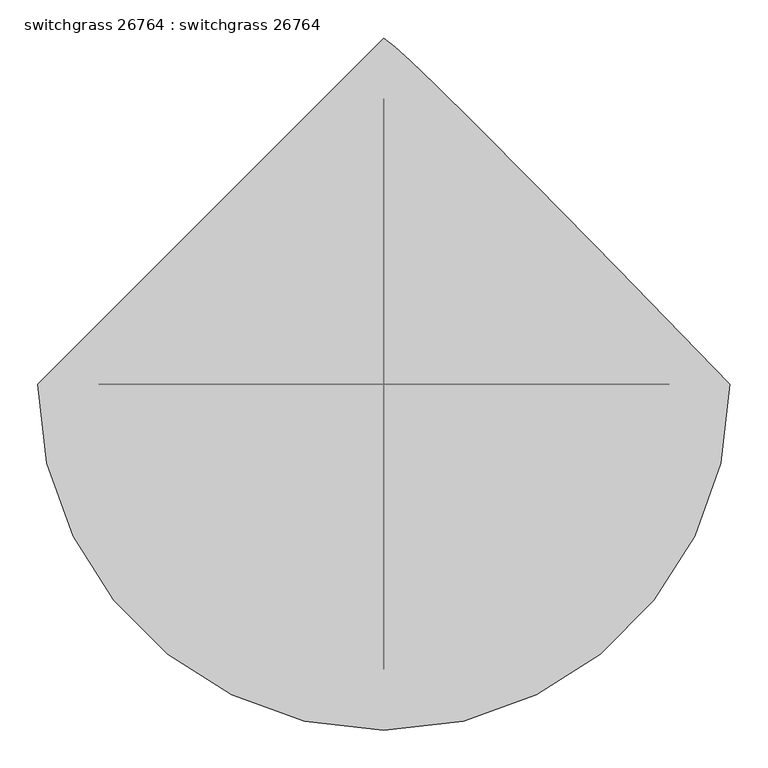
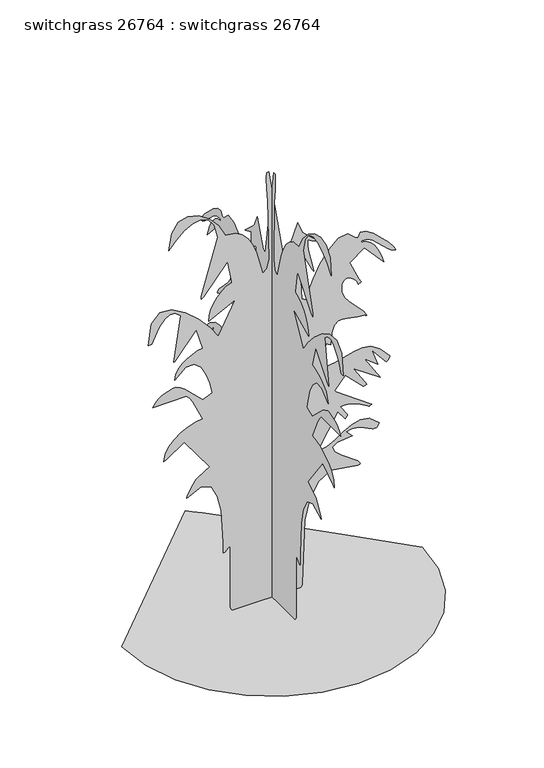
"""IFC4 building model written with IfcOpenShell, lengths in millimetres: proxy geometry, switchgrass 26764 : switchgrass 26764."""

from ifc_helpers import new_model, si_unit, origin, place, context, project, spatial, triangles, source, transform, mapped, element, save


def switchgrass_26764_switchgrass_26764_1323c538(model_context):
    return source(origin(), model_context, "Body", "Tessellation", [
        triangles([(-457.5348269, 0.0, 5.72e-05), (-445.4393443, -104.8366151, 5.72e-05), (-410.9893759, -201.1121793, 5.72e-05), (-356.9483794, -286.0697479, 5.72e-05), (-286.0697479, -356.9483794, 5.72e-05), (-201.1121793, -410.9893759, 5.72e-05), (-104.8366151, -445.4393443, 5.72e-05), (2e-05, -457.5348269, 5.72e-05), (104.8366151, -445.4393443, 5.72e-05), (201.1124336, -410.9893759, 5.72e-05), (286.0697479, -356.9483794, 5.72e-05), (356.9483794, -286.0697479, 5.72e-05), (410.9893759, -201.1121793, 5.72e-05), (445.4393443, -104.8366151, 5.72e-05), (457.5348269, 4e-05, 5.72e-05), (308.8459013, 152.5179615, 5.72e-05), (198.615602, 264.8099809, 5.72e-05), (120.4339824, 343.5803727, 5.72e-05), (67.8913365, 395.5334879, 5.72e-05), (34.5780016, 427.3748946, 5.72e-05), (14.0840831, 445.8076721, 5.72e-05), (-6e-05, 457.5348269, 5.72e-05), (34.93284, 5.5e-06, 1088.4574717), (36.237382, 5.5e-06, 1088.5946726), (37.9539129, 5.5e-06, 1088.9655075), (39.8896437, 5.5e-06, 1089.5065355), (41.8515379, 5.4e-06, 1090.1567139), (43.6465546, 5.4e-06, 1090.8526743), (45.0816551, 5.3e-06, 1091.5334467), (45.9643001, 5.3e-06, 1092.1353722), (79.0584374, 3e-07, 1176.7097157), (93.7670509, 2.4e-06, 1139.9381956), (141.570056, 5.1e-06, 1095.8133453), (139.9581813, 5e-06, 1096.2705122), (120.3097713, 3.5e-06, 1104.9699812), (109.4510318, 2.7e-06, 1111.5257584), (108.7718309, 3.8e-06, 1094.9344746), (110.1157441, 4.9e-06, 1079.5497305), (124.110375, 9.5e-06, 1020.4566805), (126.8614426, 1.06e-05, 1003.8832008), (124.028585, 1.03e-05, 1007.8913137), (90.0899044, 6.2e-06, 1077.4263136), (82.7355931, 6.2e-06, 1077.4263136), (90.0899044, 1.52e-05, 926.664731), (91.5981517, 1.52e-05, 926.3243448), (93.839948, 1.52e-05, 925.4277426), (96.493992, 1.53e-05, 924.1679358), (99.2384648, 1.54e-05, 922.7353924), (101.7517925, 1.55e-05, 921.3205805), (103.7124104, 1.55e-05, 920.1165842), (104.7985178, 1.56e-05, 919.30893), (110.3578079, 1.41e-05, 944.2085003), (125.3806282, 1.19e-05, 981.1629307), (147.3843723, 9.5e-06, 1022.163553), (173.8869515, 7.3e-06, 1059.1942142), (202.4055415, 5.8e-06, 1084.2512604), (230.4577718, 5.5e-06, 1089.3210817), (255.5618354, 6.8e-06, 1066.3950829), (262.9151293, 6.8e-06, 1066.3950829), (269.3514915, 6.1e-06, 1080.2456909), (285.9199024, 6.4e-06, 1077.2713085), (308.5106383, 7.4e-06, 1062.4834757), (355.3227882, 1.03e-05, 1017.5331671), (371.3222114, 1.13e-05, 997.3934807), (376.9076989, 1.17e-05, 985.4987125), (366.3362148, 1.13e-05, 987.6501074), (353.3212752, 1.07e-05, 997.467168), (306.0061764, 8.2e-06, 1041.5234179), (289.6028898, 7.7e-06, 1050.6166128), (273.9463418, 7.7e-06, 1051.6859516), (270.2709666, 7.9e-06, 1048.0105946), (286.0621357, 8.1e-06, 1044.6704641), (300.011793, 8.7e-06, 1035.6788618), (312.0590046, 9.4e-06, 1022.5750105), (322.1529742, 1.04e-05, 1006.8905754), (330.2352207, 1.14e-05, 990.169721), (336.2473901, 1.23e-05, 973.9468014), (340.1361425, 1.32e-05, 959.7583506), (281.3021792, 9.2e-06, 1025.9481331), (237.175821, 1.12e-05, 992.8519701), (237.8959079, 1.14e-05, 989.6693882), (264.7083701, 1.53e-05, 931.0716568), (271.2971213, 1.6e-05, 919.3597263), (262.201401, 1.58e-05, 915.7986065), (257.5227259, 1.51e-05, 925.7833895), (250.3543407, 1.46e-05, 934.7876364), (241.7117542, 1.42e-05, 941.820928), (232.6099115, 1.39e-05, 945.8899384), (224.0638488, 1.4e-05, 946.014422), (217.0887659, 1.43e-05, 941.1985823), (212.6996442, 1.49e-05, 930.4569414), (212.5952538, 1.63e-05, 907.9474869), (220.1395426, 1.74e-05, 888.4809425), (232.934274, 1.85e-05, 871.1581627), (278.8409195, 2.13e-05, 823.0557209), (288.6554731, 2.24e-05, 805.3188675), (284.9775544, 2.24e-05, 805.3188675), (284.9775544, 2.22e-05, 808.9968407), (261.1244319, 2.2e-05, 811.3030952), (219.0793602, 2.16e-05, 819.2355326), (202.3661725, 2.16e-05, 817.8461552), (189.5122514, 2.22e-05, 808.2093887), (181.2572684, 2.35e-05, 786.8149824), (178.341349, 2.57e-05, 750.1603157), (163.6327264, 2.52e-05, 757.5161167), (156.2784152, 2.96e-05, 683.9730766), (191.325313, 2.94e-05, 687.4935013), (248.5903132, 2.85e-05, 703.0763437), (274.1444584, 2.83e-05, 706.7441431), (299.8746466, 2.85e-05, 702.0628881), (327.443785, 2.96e-05, 684.8417009), (358.5206308, 3.16e-05, 650.8794571), (358.1040865, 3.17e-05, 648.5070728), (356.9788645, 3.19e-05, 645.8020054), (355.3380126, 3.21e-05, 643.0156202), (353.374615, 3.22e-05, 640.4019716), (351.2841903, 3.24e-05, 638.2225988), (349.2598226, 3.24e-05, 636.7265419), (347.4894364, 3.25e-05, 636.1703259), (303.3646043, 2.94e-05, 687.6509771), (321.6983145, 3.25e-05, 637.1100941), (281.4164709, 3.05e-05, 668.6899252), (329.1049481, 3.51e-05, 592.0454756), (248.2070336, 3.18e-05, 647.2014839), (249.7422051, 3.2e-05, 643.9071356), (282.1810136, 3.5e-05, 593.8082314), (288.6554731, 3.55e-05, 584.6896382), (287.7740952, 3.56e-05, 584.486453), (278.9298131, 3.57e-05, 581.2174664), (277.6242605, 3.58e-05, 581.0117014), (222.4671985, 3.25e-05, 636.1703259), (189.3728159, 3.49e-05, 595.7208326), (303.3646043, 3.97e-05, 514.8244623), (302.6254598, 3.97e-05, 514.6872977), (301.5739069, 3.97e-05, 514.3164628), (300.3369185, 3.98e-05, 513.7754348), (299.0364347, 3.98e-05, 513.1252201), (297.7994644, 3.98e-05, 512.4292597), (296.7479115, 3.99e-05, 511.7485236), (296.008767, 3.99e-05, 511.1465618), (285.8436898, 3.91e-05, 517.9918562), (258.9959281, 3.82e-05, 530.9178841), (230.2492453, 3.8e-05, 539.6935839), (217.7123288, 3.81e-05, 541.3522036), (207.7585759, 3.82e-05, 540.564788), (229.8212554, 4.01e-05, 507.4711684), (229.5405858, 4.03e-05, 505.7007823), (228.7854538, 4.04e-05, 503.6738711), (227.6866473, 4.05e-05, 501.5834464), (226.3747361, 4.06e-05, 499.6225923), (224.9802718, 4.07e-05, 497.9817404), (223.6343329, 4.08e-05, 496.8565184), (222.4671985, 4.08e-05, 496.4374306), (200.4042828, 3.9e-05, 525.8556567), (137.8929095, 4.54e-05, 419.2189608), (166.0807783, 4.51e-05, 424.9746051), (192.3560459, 4.44e-05, 438.7921846), (217.6356256, 4.35e-05, 455.4799742), (242.8367037, 4.28e-05, 469.858893), (268.8765023, 4.25e-05, 476.7397593), (296.6716989, 4.29e-05, 470.9409127), (327.1389708, 4.44e-05, 447.2757874), (326.9992627, 4.44e-05, 446.6026817), (318.6350567, 4.45e-05, 435.0634515), (318.0737174, 4.45e-05, 433.928092), (304.8454187, 4.44e-05, 435.7644988), (292.8515469, 4.41e-05, 440.3060094), (269.6842292, 4.35e-05, 451.6369311), (257.0629792, 4.32e-05, 455.5028289), (242.7904856, 4.32e-05, 456.2140137), (226.1443541, 4.34e-05, 452.3125803), (244.5298779, 4.45e-05, 433.928092), (198.3082625, 4.53e-05, 429.3560964), (183.5841612, 4.73e-05, 417.3698367), (191.3966749, 5e-05, 400.5525129), (212.7859943, 5.3e-05, 381.4872886), (260.4513443, 5.75e-05, 346.9661762), (268.8053947, 5.81e-05, 336.6766517), (266.5219404, 5.8e-05, 334.0198371), (261.1066641, 5.8e-05, 333.3340141), (178.1579663, 6e-05, 346.4759809), (140.1265758, 6.16e-05, 322.2393062), (114.9013532, 6.35e-05, 274.7464384), (99.9910624, 6.53e-05, 212.9973368), (92.4787665, 7.02e-05, 12.5836557), (91.8127825, 7.03e-05, 8.321819), (90.5290672, 7.04e-05, 4.9722738), (88.4818266, 7.04e-05, 2.3959441), (85.5242583, 7.04e-05, 0.4537325), (-118.3633693, 7.08e-05, 2.4e-05), (-122.0969169, 7.09e-05, 2.3783469), (-124.6485962, 7.1e-05, 5.1976728), (-126.2274606, 7.11e-05, 8.3395482), (-127.0420366, 7.12e-05, 11.6852833), (-127.3018772, 7.12e-05, 15.1165158), (-126.9912402, 7.13e-05, 21.7608447), (-126.8614426, 5.81e-05, 205.9442608), (-129.3712185, 5.82e-05, 207.0623793), (-132.5175108, 5.83e-05, 205.407811), (-143.2413748, 5.85e-05, 195.0563171), (-146.3985949, 5.86e-05, 193.5589884), (-148.9243673, 5.88e-05, 194.9127939), (-148.7935613, 5.68e-05, 227.8207598), (-154.894379, 5.06e-05, 331.9700349), (-165.8895291, 4.76e-05, 382.8233262), (-185.3575813, 4.54e-05, 419.2723005), (-215.6798221, 4.47e-05, 431.1264825), (-259.2397541, 4.61e-05, 408.1877664), (-259.6156759, 4.59e-05, 410.1283092), (-257.8935608, 4.56e-05, 415.3124405), (-244.622078, 4.41e-05, 440.6336783), (-233.4986654, 4.32e-05, 455.9905171), (-232.2906359, 4.31e-05, 458.4568274), (-228.0976142, 4.28e-05, 462.3633476), (-205.3272926, 4.19e-05, 477.5550802), (-189.3728159, 4.15e-05, 485.4061998), (-266.593048, 3.51e-05, 592.0454756), (-321.7491108, 3.73e-05, 555.2739192), (-329.1049481, 3.75e-05, 551.5960187), (-325.1247405, 3.62e-05, 573.5644452), (-314.238341, 3.5e-05, 593.5542134), (-298.0255225, 3.4e-05, 611.0903887), (-278.058609, 3.31e-05, 625.6979273), (-255.9199894, 3.24e-05, 636.9018219), (-233.1864933, 3.2e-05, 644.2271742), (-211.4357316, 3.18e-05, 647.2014839), (-213.7123368, 3.13e-05, 653.8029705), (-240.9860717, 2.74e-05, 712.3753401), (-250.6378082, 2.7e-05, 726.9625311), (-260.7383544, 2.74e-05, 738.2883659), (-362.9504113, 3.12e-05, 737.0260157), (-353.9791203, 3.02e-05, 749.4745291), (-345.6987391, 2.91e-05, 758.1181149), (-337.7028245, 2.78e-05, 763.9169615), (-329.5900566, 2.65e-05, 767.8437567), (-300.461384, 2.23e-05, 778.026638), (-293.1055467, 2.23e-05, 778.026638), (-278.8536186, 2.33e-05, 770.8663919), (-266.2755528, 2.42e-05, 762.6672558), (-211.4357316, 2.81e-05, 709.7133659), (-182.0185046, 2.74e-05, 720.7445967), (-189.8899537, 2.53e-05, 755.5907982), (-200.3534683, 2.34e-05, 786.4390606), (-215.7232605, 2.17e-05, 814.9480036), (-236.4161108, 2.06e-05, 832.6416183), (-262.8490904, 2.07e-05, 831.0515991), (-295.4347286, 2.24e-05, 801.707024), (-292.5975471, 2.14e-05, 818.2246204), (-284.8327776, 2.06e-05, 832.9972652), (-273.265624, 1.99e-05, 845.8724968), (-259.0162394, 1.93e-05, 856.6852816), (-243.2146603, 1.88e-05, 865.2806145), (-226.9795139, 1.84e-05, 871.5010923), (-211.4357316, 1.82e-05, 875.1840797), (-229.8215097, 1.43e-05, 941.3738623), (-296.0113104, 1.91e-05, 860.4749485), (-299.6866857, 1.91e-05, 860.4749485), (-277.7029984, 1e-05, 1003.3269121), (-294.71337, 9.2e-06, 1017.2435772), (-311.0531794, 9.3e-06, 1017.8481188), (-326.2398251, 9.9e-06, 1008.5745569), (-339.7957927, 1.1e-05, 992.857057), (-351.2410243, 1.22e-05, 974.1270956), (-365.8764682, 1.43e-05, 941.3738623), (-376.9076989, 1.43e-05, 941.3738623), (-367.2226796, 1.04e-05, 1007.1064779), (-341.7211112, 8.7e-06, 1034.375889), (-305.7369704, 8.9e-06, 1031.8511158), (-264.604234, 1.03e-05, 1008.203722), (-223.6538811, 1.25e-05, 972.1078148), (-188.2191436, 1.48e-05, 932.229871), (-163.6329808, 1.69e-05, 897.2464685), (-112.1528291, 1.1e-05, 996.5298706), (-193.0499715, 1.34e-05, 956.0804501), (-191.1398955, 1.24e-05, 973.1822405), (-185.7319771, 1.13e-05, 990.7996971), (-177.3111248, 1.03e-05, 1008.0386158), (-166.3611936, 9.4e-06, 1024.0076265), (-153.3675827, 8.5e-06, 1037.8124525), (-138.8136563, 7.9e-06, 1048.5617237), (-123.1842869, 7.5e-06, 1055.3638521), (-122.7161651, 7.3e-06, 1058.0105656), (-134.2157538, 3.3e-06, 1125.2290644), (-138.2424067, 3.4e-06, 1124.548292), (-207.9053874, 8.4e-06, 1039.524412), (-215.1128872, 8.8e-06, 1033.3014633), (-214.9937629, 6.5e-06, 1043.3674913), (-165.5864953, -2.1e-06, 1216.2397156), (-176.4513299, -4.6e-06, 1258.3223213), (-194.0382833, -6.1e-06, 1282.2669353), (-216.3737477, -6.6e-06, 1290.7911243), (-241.4831526, -6.4e-06, 1286.6001011), (-267.3931445, -5.6e-06, 1272.4143391), (-292.1276449, -4.3e-06, 1250.938615), (-313.7150808, -2.8e-06, 1224.8909317), (-305.8919028, -5.9e-06, 1277.1868675), (-285.2950496, -7.5e-06, 1305.4849949), (-256.2374846, -8e-06, 1313.3996281), (-223.0242321, -7.4e-06, 1304.5427559), (-189.9694546, -6.1e-06, 1282.5285473), (-161.3812832, -4.2e-06, 1250.9716072), (-141.570056, -1.9e-06, 1213.4812357), (-111.003735, -1.7e-06, 1210.2630455), (-90.0827918, -1e-06, 1197.192259), (-72.9868286, 2e-07, 1178.0406664), (-59.2218167, 1.6e-06, 1154.5431181), (-48.2927191, 3.1e-06, 1128.4294504), (-27.578531, 7.7e-06, 1051.6859516), (-15.6259369, 7e-06, 1062.9330849), (-8.9939533, 5.3e-06, 1092.3284563), (-12.8700152, -6.1e-06, 1283.3463753), (-14.1246216, -5.9e-06, 1292.5767712), (-15.1875847, -6.3e-06, 1303.493692), (-16.0281459, -7e-06, 1315.7644547), (-16.6151389, -8.1e-06, 1329.0460567), (-16.9180092, -9.2e-06, 1343.0058151), (-16.9057404, -1.04e-05, 1357.3034889), (-16.5471686, -1.14e-05, 1371.5986919), (-9.1928857, -1.14e-05, 1371.5986919), (-3.16e-05, 34.93284, 1088.4574717), (-3.16e-05, 36.237382, 1088.5946726), (-3.16e-05, 37.9539129, 1088.9655075), (-3.16e-05, 39.8896437, 1089.509079), (-3.16e-05, 41.8515379, 1090.1567139), (-3.16e-05, 43.6465546, 1090.8552177), (-3.16e-05, 45.0819049, 1091.5334467), (-3.16e-05, 45.9643001, 1092.1353722), (-3.16e-05, 79.0586918, 1176.7097157), (-3.16e-05, 93.7673053, 1139.9381956), (-3.16e-05, 141.570056, 1095.8133453), (-3.15e-05, 139.9581813, 1096.2705122), (-3.05e-05, 120.3097713, 1104.9699812), (-3.01e-05, 109.4512861, 1111.5257584), (-3.02e-05, 108.7720852, 1094.9344746), (-3.04e-05, 110.1157441, 1079.5497305), (-3.15e-05, 124.1106294, 1020.4566805), (-3.16e-05, 126.8614426, 1003.8832008), (-3.16e-05, 124.028585, 1007.8913137), (-3.16e-05, 90.0901496, 1077.4263136), (-3.16e-05, 82.7358474, 1077.4263136), (-3.16e-05, 90.0901496, 926.664731), (-3.16e-05, 91.5981517, 926.3243448), (-3.16e-05, 93.8402023, 925.4277426), (-3.16e-05, 96.493992, 924.1679358), (-3.16e-05, 99.2387191, 922.7353924), (-3.16e-05, 101.7517925, 921.3205805), (-3.16e-05, 103.7124104, 920.1165842), (-3.16e-05, 104.7985178, 919.30893), (-3.16e-05, 110.3578079, 944.2085003), (-3.16e-05, 125.3806282, 981.1629307), (-3.16e-05, 147.3846266, 1022.163553), (-3.16e-05, 173.8872059, 1059.1942142), (-3.16e-05, 202.4055415, 1084.2512604), (-3.16e-05, 230.4580261, 1089.3210817), (-3.16e-05, 255.5618354, 1066.3950829), (-3.16e-05, 262.9151293, 1066.3950829), (-3.16e-05, 269.3514915, 1080.2456909), (-3.18e-05, 285.9199024, 1077.2713085), (-3.19e-05, 308.5106383, 1062.4834757), (-3.21e-05, 355.3227882, 1017.5331671), (-3.19e-05, 371.3222114, 997.3934807), (-3.16e-05, 376.9076989, 985.4987125), (-3.14e-05, 366.3362148, 987.6501074), (-3.13e-05, 353.3212752, 997.467168), (-3.14e-05, 306.0061764, 1041.5234179), (-3.15e-05, 289.6028898, 1050.6166128), (-3.16e-05, 273.9463418, 1051.6859516), (-3.16e-05, 270.2709666, 1048.0105946), (-3.16e-05, 286.0621357, 1044.6704641), (-3.16e-05, 300.011793, 1035.6788618), (-3.16e-05, 312.0590046, 1022.5750105), (-3.16e-05, 322.1529742, 1006.8905754), (-3.16e-05, 330.2352207, 990.169721), (-3.16e-05, 336.2473901, 973.9468014), (-3.16e-05, 340.1361425, 959.7583506), (-3.16e-05, 281.3021792, 1025.9481331), (-3.16e-05, 237.175821, 992.8519701), (-3.16e-05, 237.8959079, 989.6693882), (-3.19e-05, 264.7083701, 931.0716568), (-3.19e-05, 271.2971213, 919.3597263), (-3.16e-05, 262.201401, 915.7986065), (-3.15e-05, 257.5227259, 925.7833895), (-3.15e-05, 250.3543407, 934.7876364), (-3.15e-05, 241.7117542, 941.820928), (-3.15e-05, 232.6099115, 945.8924818), (-3.15e-05, 224.0641032, 946.014422), (-3.15e-05, 217.0887659, 941.1985823), (-3.16e-05, 212.6996442, 930.4569414), (-3.16e-05, 212.5955081, 907.9474869), (-3.16e-05, 220.1397969, 888.4809425), (-3.16e-05, 232.934274, 871.1581627), (-3.16e-05, 278.8409195, 823.0557209), (-3.16e-05, 288.6554731, 805.3188675), (-3.16e-05, 284.9775544, 805.3188675), (-3.16e-05, 284.9775544, 808.9968407), (-3.16e-05, 261.1244319, 811.3030952), (-3.16e-05, 219.0796145, 819.2355326), (-3.16e-05, 202.3661725, 817.8461552), (-3.16e-05, 189.5122514, 808.2093887), (-3.16e-05, 181.2575227, 786.8149824), (-3.16e-05, 178.3416033, 750.1603157), (-3.16e-05, 163.6329808, 757.5161167), (-3.16e-05, 156.2786695, 683.9730766), (-3.16e-05, 191.325313, 687.4935013), (-3.16e-05, 248.5905676, 703.0763437), (-3.16e-05, 274.1444584, 706.7441431), (-3.16e-05, 299.8746466, 702.0628881), (-3.16e-05, 327.443785, 684.8417009), (-3.16e-05, 358.5206308, 650.8794571), (-3.16e-05, 358.1040865, 648.5070728), (-3.16e-05, 356.9788645, 645.8020054), (-3.16e-05, 355.3380126, 643.0156202), (-3.16e-05, 353.374615, 640.4019716), (-3.16e-05, 351.2841903, 638.2225988), (-3.16e-05, 349.2598226, 636.7265419), (-3.16e-05, 347.4894364, 636.1703259), (-3.16e-05, 303.3646043, 687.6509771), (-3.17e-05, 321.6983145, 637.1100941), (-3.16e-05, 281.4164709, 668.6899252), (-3.16e-05, 329.1049481, 592.0454756), (-3.16e-05, 248.2072879, 647.2014839), (-3.16e-05, 249.7422051, 643.9071356), (-3.16e-05, 282.1810136, 593.8082314), (-3.16e-05, 288.6554731, 584.6896382), (-3.16e-05, 287.7740952, 584.486453), (-3.16e-05, 278.9298131, 581.2174664), (-3.16e-05, 277.6242605, 581.0117014), (-3.16e-05, 222.4671985, 636.1703259), (-3.16e-05, 189.3728159, 595.7208326), (-3.16e-05, 303.3646043, 514.8244623), (-3.16e-05, 302.6254598, 514.6872977), (-3.16e-05, 301.5739069, 514.3164628), (-3.16e-05, 300.3369185, 513.7754348), (-3.16e-05, 299.0364347, 513.1252201), (-3.16e-05, 297.7994644, 512.4292597), (-3.16e-05, 296.7479115, 511.7485236), (-3.16e-05, 296.0113104, 511.1465618), (-3.12e-05, 285.8436898, 517.9918562), (-3.1e-05, 258.9959281, 530.9178841), (-3.13e-05, 230.2494996, 539.6935839), (-3.15e-05, 217.7125832, 541.3522036), (-3.16e-05, 207.7585759, 540.564788), (-3.16e-05, 229.8215097, 507.4711684), (-3.16e-05, 229.5408401, 505.7007823), (-3.16e-05, 228.7857081, 503.6738711), (-3.16e-05, 227.6866473, 501.5834464), (-3.16e-05, 226.3747361, 499.6225923), (-3.16e-05, 224.9805262, 497.9817404), (-3.16e-05, 223.6343329, 496.8565184), (-3.16e-05, 222.4671985, 496.4374306), (-3.16e-05, 200.4042828, 525.8556567), (-3.16e-05, 137.8929095, 419.2189608), (-3.16e-05, 166.0807783, 424.9771485), (-3.17e-05, 192.3560459, 438.7921846), (-3.18e-05, 217.63588, 455.4799742), (-3.19e-05, 242.8367037, 469.858893), (-3.21e-05, 268.8765023, 476.7397593), (-3.21e-05, 296.6716989, 470.9409127), (-3.22e-05, 327.1389708, 447.2757874), (-3.21e-05, 326.9992627, 446.6026817), (-3.16e-05, 318.6350567, 435.0634515), (-3.16e-05, 318.0737174, 433.928092), (-3.16e-05, 304.8454187, 435.7644988), (-3.16e-05, 292.8540904, 440.3060094), (-3.16e-05, 269.6842292, 451.6369311), (-3.16e-05, 257.0629792, 455.5028289), (-3.16e-05, 242.7904856, 456.2140137), (-3.16e-05, 226.1443541, 452.3125803), (-3.16e-05, 244.5301323, 433.928092), (-3.21e-05, 198.3082625, 429.3560964), (-3.33e-05, 183.5841612, 417.3698367), (-3.51e-05, 191.3969293, 400.5525129), (-3.69e-05, 212.7862487, 381.4872886), (-3.94e-05, 260.4513443, 346.9661762), (-3.94e-05, 268.8053947, 336.6766517), (-3.91e-05, 266.5219404, 334.0198371), (-3.91e-05, 261.1066641, 333.3340141), (-4.18e-05, 178.1579663, 346.4759809), (-4.2e-05, 140.1265758, 322.2393062), (-4.1e-05, 114.9013532, 274.7464384), (-3.92e-05, 99.9910624, 212.9973368), (-3.21e-05, 92.4787665, 12.5836296), (-3.2e-05, 91.8127825, 8.3217934), (-3.19e-05, 90.5293216, 4.9722483), (-3.18e-05, 88.4818266, 2.3959185), (-3.16e-05, 85.5242583, 0.4537071), (-3.19e-05, -118.3631241, 0.0), (-3.22e-05, -122.0966625, 2.378324), (-3.24e-05, -124.6483418, 5.1976479), (-3.27e-05, -126.2272062, 8.3395226), (-3.3e-05, -127.0420366, 11.6852833), (-3.33e-05, -127.3018772, 15.1164896), (-3.38e-05, -126.9912402, 21.7608197), (-3.16e-05, -126.8614426, 205.9442608), (-3.17e-05, -129.3709642, 207.062125), (-3.17e-05, -132.5175108, 205.407811), (-3.13e-05, -143.2413748, 195.0563171), (-3.13e-05, -146.3985949, 193.5589884), (-3.16e-05, -148.924113, 194.9127939), (-3.16e-05, -148.7935613, 227.8207598), (-3.16e-05, -154.8941247, 331.9700349), (-3.16e-05, -165.8895291, 382.8233262), (-3.16e-05, -185.357327, 419.274844), (-3.16e-05, -215.6798221, 431.1264825), (-3.16e-05, -259.2397541, 408.1877664), (-3.16e-05, -259.6156759, 410.1283092), (-3.16e-05, -257.8935608, 415.3124405), (-3.16e-05, -244.6218236, 440.6336783), (-3.16e-05, -233.498411, 455.9905171), (-3.16e-05, -232.2906359, 458.4568274), (-3.16e-05, -228.0976142, 462.3658911), (-3.16e-05, -205.3272926, 477.5550802), (-3.16e-05, -189.3728159, 485.4061998), (-3.16e-05, -266.593048, 592.0454756), (-3.16e-05, -321.7491108, 555.2739192), (-3.16e-05, -329.1049481, 551.5960187), (-3.16e-05, -325.1247405, 573.5644452), (-3.16e-05, -314.238341, 593.5542134), (-3.16e-05, -298.0229791, 611.0903887), (-3.16e-05, -278.058609, 625.6979273), (-3.16e-05, -255.9199894, 636.9018219), (-3.16e-05, -233.186239, 644.2271742), (-3.16e-05, -211.4357316, 647.2014839), (-3.14e-05, -213.7123368, 653.8029705), (-3.1e-05, -240.9858174, 712.3753401), (-3.15e-05, -250.6378082, 726.9625311), (-3.26e-05, -260.7383544, 738.2883659), (-3.63e-05, -362.9504113, 737.0260157), (-3.61e-05, -353.9765768, 749.4745291), (-3.54e-05, -345.6987391, 758.1181149), (-3.45e-05, -337.7028245, 763.9169615), (-3.34e-05, -329.5900566, 767.8437567), (-2.99e-05, -300.461384, 778.026638), (-2.99e-05, -293.1055467, 778.026638), (-3.04e-05, -278.8536186, 770.8663919), (-3.08e-05, -266.2730093, 762.6672558), (-3.16e-05, -211.4357316, 709.7133659), (-3.16e-05, -182.0185046, 720.7445967), (-3.15e-05, -189.8899537, 755.5907982), (-3.15e-05, -200.353214, 786.4390606), (-3.15e-05, -215.7232605, 814.9480036), (-3.14e-05, -236.4161108, 832.6416183), (-3.14e-05, -262.8465652, 831.0515991), (-3.14e-05, -295.4347286, 801.707024), (-3.14e-05, -292.5975471, 818.2246204), (-3.14e-05, -284.8327776, 832.9972652), (-3.15e-05, -273.265624, 845.8724968), (-3.15e-05, -259.0162394, 856.6852816), (-3.15e-05, -243.2146603, 865.2806145), (-3.16e-05, -226.9795139, 871.5010923), (-3.16e-05, -211.4357316, 875.1840797), (-3.16e-05, -229.8212554, 941.3738623), (-3.16e-05, -296.008767, 860.4749485), (-3.16e-05, -299.6866857, 860.4749485), (-3.1e-05, -277.7029984, 1003.3269121), (-3.1e-05, -294.71337, 1017.2435772), (-3.11e-05, -311.0531794, 1017.8481188), (-3.12e-05, -326.2398251, 1008.5745569), (-3.13e-05, -339.7957927, 992.857057), (-3.14e-05, -351.2384809, 974.1270956), (-3.16e-05, -365.8764682, 941.3738623), (-3.16e-05, -376.9076989, 941.3738623), (-3.16e-05, -367.2226796, 1007.1064779), (-3.16e-05, -341.7211112, 1034.375889), (-3.16e-05, -305.7369704, 1031.8511158), (-3.16e-05, -264.604234, 1008.203722), (-3.16e-05, -223.6538811, 972.1078148), (-3.16e-05, -188.2191436, 932.229871), (-3.16e-05, -163.6327264, 897.2464685), (-3.16e-05, -112.1528291, 996.5298706), (-3.16e-05, -193.0499715, 956.0804501), (-3.16e-05, -191.1396412, 973.1822405), (-3.16e-05, -185.7317227, 990.7996971), (-3.16e-05, -177.3108705, 1008.0386158), (-3.16e-05, -166.3611936, 1024.0076265), (-3.16e-05, -153.3673283, 1037.8124525), (-3.16e-05, -138.813402, 1048.5617237), (-3.16e-05, -123.1842869, 1055.3638521), (-3.16e-05, -122.7159107, 1058.0105656), (-3.16e-05, -134.2157538, 1125.2290644), (-3.16e-05, -138.2424067, 1124.548292), (-3.16e-05, -207.9053874, 1039.524412), (-3.16e-05, -215.1128872, 1033.3014633), (-2.99e-05, -214.9935086, 1043.3674913), (-3.16e-05, -165.5864953, 1216.2397156), (-3.16e-05, -176.4510756, 1258.3223213), (-3.15e-05, -194.0382833, 1282.2669353), (-3.15e-05, -216.3737477, 1290.7911243), (-3.15e-05, -241.4828982, 1286.6001011), (-3.14e-05, -267.3931445, 1272.4143391), (-3.14e-05, -292.1276449, 1250.938615), (-3.14e-05, -313.7150808, 1224.8909317), (-3.14e-05, -305.8919028, 1277.1868675), (-3.14e-05, -285.2950496, 1305.4849949), (-3.15e-05, -256.2349411, 1313.3996281), (-3.15e-05, -223.0242321, 1304.5427559), (-3.15e-05, -189.9694546, 1282.5285473), (-3.16e-05, -161.3812832, 1250.9716072), (-3.16e-05, -141.570056, 1213.4812357), (-3.16e-05, -111.003735, 1210.2630455), (-3.16e-05, -90.0825374, 1197.192259), (-3.16e-05, -72.9865742, 1178.0432098), (-3.16e-05, -59.2215669, 1154.5431181), (-3.16e-05, -48.2927191, 1128.4294504), (-3.16e-05, -27.578531, 1051.6859516), (-3.16e-05, -15.6258108, 1062.9330849), (-3.16e-05, -8.9938517, 1092.3284563), (-3.16e-05, -12.869888, 1283.3463753), (-3.23e-05, -14.1245194, 1292.5767712), (-3.26e-05, -15.1874576, 1303.493692), (-3.26e-05, -16.0280449, 1315.7644547), (-3.23e-05, -16.6150378, 1329.0460567), (-3.2e-05, -16.917907, 1343.0058151), (-3.17e-05, -16.9056394, 1357.3034889), (-3.16e-05, -16.5470675, 1371.5986919), (-3.16e-05, -9.1927591, 1371.5986919)], [[21, 22, 1], [20, 21, 1], [19, 20, 1], [18, 19, 1], [17, 18, 1], [17, 1, 2], [17, 2, 3], [17, 3, 4], [16, 17, 4], [16, 4, 5], [16, 5, 6], [16, 6, 7], [16, 7, 8], [16, 8, 9], [16, 9, 10], [16, 10, 11], [16, 11, 12], [15, 16, 12], [14, 15, 12], [13, 14, 12], [122, 123, 124], [39, 40, 41], [77, 78, 79], [76, 77, 79], [32, 33, 34], [32, 34, 35], [32, 35, 36], [75, 76, 79], [294, 295, 296], [120, 121, 122], [74, 75, 79], [246, 247, 248], [246, 248, 249], [73, 74, 79], [30, 31, 32], [132, 133, 134], [285, 286, 287], [171, 172, 173], [246, 249, 250], [218, 219, 220], [64, 65, 66], [230, 231, 232], [230, 232, 233], [230, 233, 234], [230, 234, 235], [132, 134, 135], [230, 235, 236], [230, 236, 237], [230, 237, 238], [230, 238, 239], [273, 274, 275], [273, 275, 276], [273, 276, 277], [132, 135, 136], [72, 73, 79], [132, 136, 137], [273, 277, 278], [132, 137, 138], [217, 218, 220], [217, 220, 221], [217, 221, 222], [217, 222, 223], [126, 127, 128], [103, 104, 105], [229, 230, 239], [229, 239, 240], [132, 138, 139], [207, 208, 209], [207, 209, 210], [207, 210, 211], [273, 278, 279], [30, 32, 36], [30, 36, 37], [228, 229, 240], [293, 294, 296], [293, 296, 297], [293, 297, 298], [292, 293, 298], [292, 298, 299], [291, 292, 299], [291, 299, 300], [290, 291, 300], [289, 290, 300], [289, 300, 301], [288, 289, 301], [288, 301, 302], [132, 139, 140], [132, 140, 141], [132, 141, 142], [132, 142, 143], [132, 143, 144], [132, 144, 145], [64, 66, 67], [63, 64, 67], [256, 257, 258], [255, 256, 258], [273, 279, 280], [264, 265, 266], [263, 264, 266], [262, 263, 266], [262, 266, 267], [261, 262, 267], [261, 267, 268], [260, 261, 268], [259, 260, 268], [259, 268, 269], [258, 259, 269], [255, 258, 269], [255, 269, 270], [255, 270, 271], [254, 255, 271], [254, 271, 272], [82, 83, 84], [82, 84, 85], [273, 280, 281], [71, 72, 79], [63, 67, 68], [62, 63, 68], [62, 68, 69], [61, 62, 69], [61, 69, 70], [60, 61, 70], [59, 60, 70], [207, 211, 212], [96, 97, 98], [95, 96, 98], [95, 98, 99], [317, 318, 319], [317, 319, 23], [316, 317, 23], [315, 316, 23], [314, 315, 23], [313, 314, 23], [312, 313, 23], [311, 312, 23], [310, 311, 23], [246, 250, 251], [245, 246, 251], [245, 251, 252], [82, 85, 86], [82, 86, 87], [81, 82, 87], [30, 37, 38], [95, 99, 100], [39, 41, 42], [38, 39, 42], [30, 38, 42], [30, 42, 43], [81, 87, 88], [94, 95, 100], [309, 310, 23], [227, 228, 240], [217, 223, 224], [59, 70, 71], [245, 252, 253], [177, 178, 179], [177, 179, 180], [177, 180, 181], [176, 177, 181], [175, 176, 181], [71, 79, 80], [284, 285, 287], [284, 287, 288], [284, 288, 302], [284, 302, 303], [283, 284, 303], [283, 303, 304], [283, 304, 305], [283, 305, 306], [283, 306, 307], [282, 283, 307], [282, 307, 308], [281, 282, 308], [273, 281, 308], [152, 153, 154], [151, 152, 154], [150, 151, 154], [149, 150, 154], [148, 149, 154], [147, 148, 154], [146, 147, 154], [145, 146, 154], [164, 165, 166], [94, 100, 101], [58, 59, 71], [58, 71, 80], [118, 119, 120], [117, 118, 120], [116, 117, 120], [115, 116, 120], [114, 115, 120], [113, 114, 120], [112, 113, 120], [111, 112, 120], [110, 111, 120], [93, 94, 101], [109, 110, 120], [109, 120, 122], [108, 109, 122], [108, 122, 124], [107, 108, 124], [126, 128, 129], [126, 129, 130], [125, 126, 130], [125, 130, 131], [124, 125, 131], [107, 124, 131], [107, 131, 132], [106, 107, 132], [30, 43, 44], [29, 30, 44], [28, 29, 44], [27, 28, 44], [26, 27, 44], [25, 26, 44], [24, 25, 44], [23, 24, 44], [309, 23, 44], [308, 309, 44], [273, 308, 44], [272, 273, 44], [161, 162, 163], [161, 163, 164], [161, 164, 166], [161, 166, 167], [160, 161, 167], [160, 167, 168], [160, 168, 169], [159, 160, 169], [159, 169, 170], [158, 159, 170], [158, 170, 171], [158, 171, 173], [157, 158, 173], [156, 157, 173], [156, 173, 174], [81, 88, 89], [244, 245, 253], [244, 253, 254], [201, 202, 203], [200, 201, 203], [199, 200, 203], [198, 199, 203], [207, 212, 213], [207, 213, 214], [206, 207, 214], [206, 214, 215], [206, 215, 216], [57, 58, 80], [56, 57, 80], [55, 56, 80], [54, 55, 80], [53, 54, 80], [53, 80, 81], [53, 81, 89], [53, 89, 90], [52, 53, 90], [52, 90, 91], [51, 52, 91], [51, 91, 92], [51, 92, 93], [51, 93, 101], [51, 101, 102], [244, 254, 272], [243, 244, 272], [243, 272, 44], [242, 243, 44], [241, 242, 44], [217, 224, 225], [216, 217, 225], [216, 225, 226], [51, 102, 103], [51, 103, 105], [241, 44, 45], [241, 45, 46], [241, 46, 47], [241, 47, 48], [241, 48, 49], [241, 49, 50], [241, 50, 51], [241, 51, 105], [241, 105, 106], [241, 106, 132], [241, 132, 145], [241, 145, 154], [241, 154, 155], [240, 241, 155], [227, 240, 155], [226, 227, 155], [216, 226, 155], [206, 216, 155], [205, 206, 155], [204, 205, 155], [203, 204, 155], [198, 203, 155], [197, 198, 155], [175, 181, 182], [174, 175, 182], [156, 174, 182], [155, 156, 182], [197, 155, 182], [197, 182, 183], [197, 183, 184], [196, 197, 184], [196, 184, 185], [196, 185, 186], [196, 186, 187], [196, 187, 188], [196, 188, 189], [196, 189, 190], [195, 196, 190], [194, 195, 190], [194, 190, 191], [194, 191, 192], [194, 192, 193], [419, 420, 421], [336, 337, 338], [374, 375, 376], [373, 374, 376], [329, 330, 331], [329, 331, 332], [329, 332, 333], [372, 373, 376], [591, 592, 593], [417, 418, 419], [371, 372, 376], [543, 544, 545], [543, 545, 546], [370, 371, 376], [327, 328, 329], [429, 430, 431], [582, 583, 584], [468, 469, 470], [543, 546, 547], [515, 516, 517], [361, 362, 363], [527, 528, 529], [527, 529, 530], [527, 530, 531], [527, 531, 532], [429, 431, 432], [527, 532, 533], [527, 533, 534], [527, 534, 535], [527, 535, 536], [570, 571, 572], [570, 572, 573], [570, 573, 574], [429, 432, 433], [369, 370, 376], [429, 433, 434], [570, 574, 575], [429, 434, 435], [514, 515, 517], [514, 517, 518], [514, 518, 519], [514, 519, 520], [423, 424, 425], [400, 401, 402], [526, 527, 536], [526, 536, 537], [429, 435, 436], [504, 505, 506], [504, 506, 507], [504, 507, 508], [570, 575, 576], [327, 329, 333], [327, 333, 334], [525, 526, 537], [590, 591, 593], [590, 593, 594], [590, 594, 595], [589, 590, 595], [589, 595, 596], [588, 589, 596], [588, 596, 597], [587, 588, 597], [586, 587, 597], [586, 597, 598], [585, 586, 598], [585, 598, 599], [429, 436, 437], [429, 437, 438], [429, 438, 439], [429, 439, 440], [429, 440, 441], [429, 441, 442], [361, 363, 364], [360, 361, 364], [553, 554, 555], [552, 553, 555], [570, 576, 577], [561, 562, 563], [560, 561, 563], [559, 560, 563], [559, 563, 564], [558, 559, 564], [558, 564, 565], [557, 558, 565], [556, 557, 565], [556, 565, 566], [555, 556, 566], [552, 555, 566], [552, 566, 567], [552, 567, 568], [551, 552, 568], [551, 568, 569], [379, 380, 381], [379, 381, 382], [570, 577, 578], [368, 369, 376], [360, 364, 365], [359, 360, 365], [359, 365, 366], [358, 359, 366], [358, 366, 367], [357, 358, 367], [356, 357, 367], [504, 508, 509], [393, 394, 395], [392, 393, 395], [392, 395, 396], [614, 615, 616], [614, 616, 320], [613, 614, 320], [612, 613, 320], [611, 612, 320], [610, 611, 320], [609, 610, 320], [608, 609, 320], [607, 608, 320], [543, 547, 548], [542, 543, 548], [542, 548, 549], [379, 382, 383], [379, 383, 384], [378, 379, 384], [327, 334, 335], [392, 396, 397], [336, 338, 339], [335, 336, 339], [327, 335, 339], [327, 339, 340], [378, 384, 385], [391, 392, 397], [606, 607, 320], [524, 525, 537], [514, 520, 521], [356, 367, 368], [542, 549, 550], [474, 475, 476], [474, 476, 477], [474, 477, 478], [473, 474, 478], [472, 473, 478], [368, 376, 377], [581, 582, 584], [581, 584, 585], [581, 585, 599], [581, 599, 600], [580, 581, 600], [580, 600, 601], [580, 601, 602], [580, 602, 603], [580, 603, 604], [579, 580, 604], [579, 604, 605], [578, 579, 605], [570, 578, 605], [449, 450, 451], [448, 449, 451], [447, 448, 451], [446, 447, 451], [445, 446, 451], [444, 445, 451], [443, 444, 451], [442, 443, 451], [461, 462, 463], [391, 397, 398], [355, 356, 368], [355, 368, 377], [415, 416, 417], [414, 415, 417], [413, 414, 417], [412, 413, 417], [411, 412, 417], [410, 411, 417], [409, 410, 417], [408, 409, 417], [407, 408, 417], [390, 391, 398], [406, 407, 417], [406, 417, 419], [405, 406, 419], [405, 419, 421], [404, 405, 421], [423, 425, 426], [423, 426, 427], [422, 423, 427], [422, 427, 428], [421, 422, 428], [404, 421, 428], [404, 428, 429], [403, 404, 429], [327, 340, 341], [326, 327, 341], [325, 326, 341], [324, 325, 341], [323, 324, 341], [322, 323, 341], [321, 322, 341], [320, 321, 341], [606, 320, 341], [605, 606, 341], [570, 605, 341], [569, 570, 341], [458, 459, 460], [458, 460, 461], [458, 461, 463], [458, 463, 464], [457, 458, 464], [457, 464, 465], [457, 465, 466], [456, 457, 466], [456, 466, 467], [455, 456, 467], [455, 467, 468], [455, 468, 470], [454, 455, 470], [453, 454, 470], [453, 470, 471], [378, 385, 386], [541, 542, 550], [541, 550, 551], [498, 499, 500], [497, 498, 500], [496, 497, 500], [495, 496, 500], [504, 509, 510], [504, 510, 511], [503, 504, 511], [503, 511, 512], [503, 512, 513], [354, 355, 377], [353, 354, 377], [352, 353, 377], [351, 352, 377], [350, 351, 377], [350, 377, 378], [350, 378, 386], [350, 386, 387], [349, 350, 387], [349, 387, 388], [348, 349, 388], [348, 388, 389], [348, 389, 390], [348, 390, 398], [348, 398, 399], [541, 551, 569], [540, 541, 569], [540, 569, 341], [539, 540, 341], [538, 539, 341], [514, 521, 522], [513, 514, 522], [513, 522, 523], [348, 399, 400], [348, 400, 402], [538, 341, 342], [538, 342, 343], [538, 343, 344], [538, 344, 345], [538, 345, 346], [538, 346, 347], [538, 347, 348], [538, 348, 402], [538, 402, 403], [538, 403, 429], [538, 429, 442], [538, 442, 451], [538, 451, 452], [537, 538, 452], [524, 537, 452], [523, 524, 452], [513, 523, 452], [503, 513, 452], [502, 503, 452], [501, 502, 452], [500, 501, 452], [495, 500, 452], [494, 495, 452], [472, 478, 479], [471, 472, 479], [453, 471, 479], [452, 453, 479], [494, 452, 479], [494, 479, 480], [494, 480, 481], [493, 494, 481], [493, 481, 482], [493, 482, 483], [493, 483, 484], [493, 484, 485], [493, 485, 486], [493, 486, 487], [492, 493, 487], [491, 492, 487], [491, 487, 488], [491, 488, 489], [491, 489, 490]], closed=False),
    ])


if __name__ == "__main__":
    model = new_model("IFC4")
    model_context = context("Model", 3, world=origin())
    ifc_project = project(units=[si_unit("LENGTHUNIT", "METRE", prefix="MILLI")], contexts=[model_context])
    site = spatial("IfcSite", under=ifc_project)
    building = spatial("IfcBuilding", under=site)
    placement = place(None, origin())
    switchgrass_26764_switchgrass_26764_shape = switchgrass_26764_switchgrass_26764_1323c538(model_context)
    element("IfcBuildingElementProxy", 1, Name="switchgrass 26764 : switchgrass 26764", ObjectType="switchgrass 26764 : switchgrass 26764", at=placement, inside=building, context=model_context, shape_type="MappedRepresentation", body=[
        mapped(switchgrass_26764_switchgrass_26764_shape, transform((0.0, 0.0, 0.0), x_axis=(1.0, 0.0, 0.0), y_axis=(0.0, 1.0, 0.0), z_axis=(0.0, 0.0, 1.0))),
    ])
    save(model, "model.ifc")

# Revit data of these elements
# Type "switchgrass 26764 : switchgrass 26764"
#   built-in parameter 1005195 = "RPC-16-FU2N-0J7X-A2JP-J000-ST1L-LVER-AU"
#   Height = 0
